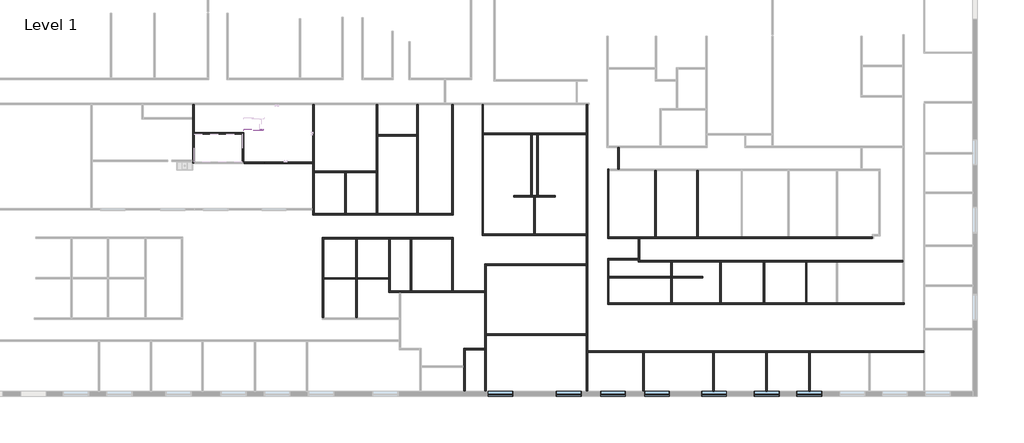
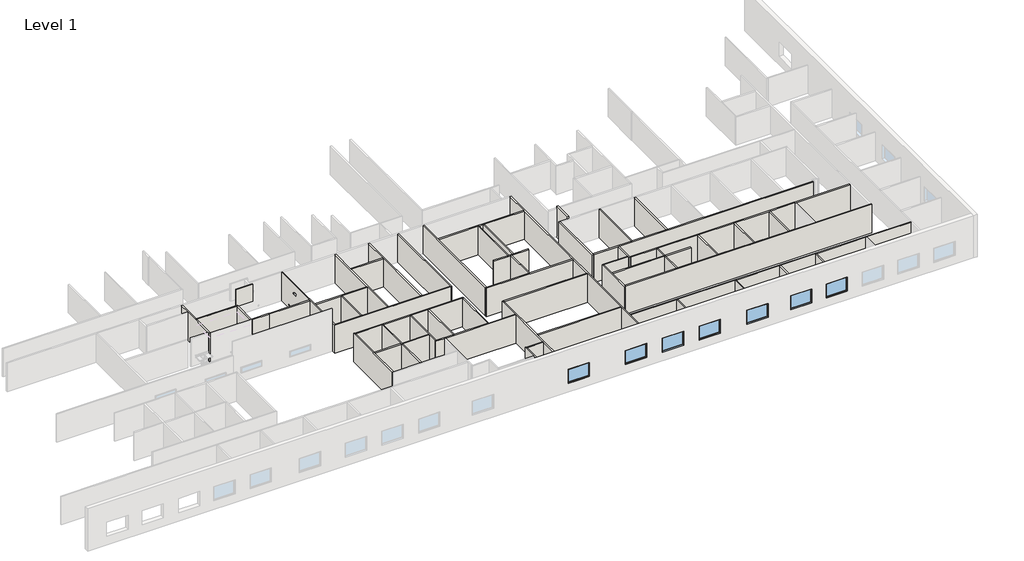
# One storey, part 2 of 4: 55 walls, 7 windows.
"""IFC4 building model written with IfcOpenShell, lengths in millimetres."""

import ifcopenshell
import ifcopenshell.guid

model = None  # the IFC model being written
_history = None  # IfcOwnerHistory: only IFC2X3 demands one
_inside = {}  # id of a spatial element -> (the spatial element, [elements in it])
_under = {}  # id of a project, library or spatial element -> (it, [spatial elements below it])
_declared = {}  # id of a project -> (the project, [libraries it declares])
_typed = {}  # id of a type object -> (the type object, [elements of that type])
_made_of = {}  # id of a material, layer set ... -> (it, [elements and type objects made of it])


def new_model(schema):
    """Start an empty IFC model of exactly this schema.

    Asked for "IFC4X3", IfcOpenShell would pick the latest addendum, in which some entities
    have other attributes; the version numbers below select the first issue.
    IFC2X3 requires an IfcOwnerHistory on every rooted entity: one is made here for all.
    """
    global model, _history
    if schema == "IFC4X3":
        model = ifcopenshell.file(schema_version=(4, 3, 0, 0))
    else:
        model = ifcopenshell.file(schema=schema)
    _inside.clear()
    _under.clear()
    _declared.clear()
    _typed.clear()
    _made_of.clear()
    _history = None
    if model.schema == "IFC2X3":
        org = make("IfcOrganization", Name="unknown")
        user = make(
            "IfcPersonAndOrganization",
            ThePerson=make("IfcPerson", FamilyName="unknown"),
            TheOrganization=org,
        )
        app = make(
            "IfcApplication",
            ApplicationDeveloper=org,
            Version="unknown",
            ApplicationFullName="unknown",
            ApplicationIdentifier="unknown",
        )
        _history = make(
            "IfcOwnerHistory",
            OwningUser=user,
            OwningApplication=app,
            ChangeAction="ADDED",
            CreationDate=0,
        )
    return model


def make(cls, **values):
    """One entity of the class cls with the attributes given. An attribute that is None is left unset."""
    return model.create_entity(
        cls, **{name: value for name, value in values.items() if value is not None}
    )


def rooted(cls, **values):
    """An entity with a GlobalId (a new one), such as an element, a storey or a relation."""
    return make(cls, GlobalId=ifcopenshell.guid.new(), OwnerHistory=_history, **values)


def si_unit(unit_type, name, prefix=None):
    """IfcSIUnit, for example si_unit("LENGTHUNIT", "METRE", prefix="MILLI")."""
    return make("IfcSIUnit", UnitType=unit_type, Prefix=prefix, Name=name)


def assignment(units):
    """IfcUnitAssignment: the units of a project."""
    return None if units is None else make("IfcUnitAssignment", Units=units)


def point(xyz):
    """IfcCartesianPoint."""
    return None if xyz is None else make("IfcCartesianPoint", Coordinates=xyz)


def direction(xyz):
    """IfcDirection."""
    return None if xyz is None else make("IfcDirection", DirectionRatios=xyz)


def frame(location, z_axis=None, x_axis=None):
    """IfcAxis2Placement3D, a coordinate frame: its origin and axes. An axis left out is left unset."""
    return make(
        "IfcAxis2Placement3D",
        Location=point(location),
        Axis=direction(z_axis),
        RefDirection=direction(x_axis),
    )


def origin():
    """The frame at (0, 0, 0) with its axes left unset."""
    return frame((0.0, 0.0, 0.0))


def origin_with_axes():
    """The frame at (0, 0, 0) with the z axis (0, 0, 1) and the x axis (1, 0, 0) written out."""
    return frame((0.0, 0.0, 0.0), z_axis=(0.0, 0.0, 1.0), x_axis=(1.0, 0.0, 0.0))


def place(relative_to, where):
    """IfcLocalPlacement: puts the frame where relative to a parent placement (None: the world)."""
    return make(
        "IfcLocalPlacement", PlacementRelTo=relative_to, RelativePlacement=where
    )


def context(
    kind, dimensions, precision=None, world=None, true_north=None, identifier=None
):
    """IfcGeometricRepresentationContext, for example the 3D "Model" context."""
    return make(
        "IfcGeometricRepresentationContext",
        ContextIdentifier=identifier,
        ContextType=kind,
        CoordinateSpaceDimension=dimensions,
        Precision=precision,
        WorldCoordinateSystem=world,
        TrueNorth=true_north,
    )


def project(units=None, contexts=None):
    """IfcProject with its units and contexts."""
    return rooted(
        "IfcProject",
        Name="project",
        RepresentationContexts=contexts,
        UnitsInContext=assignment(units),
    )


def spatial(cls, under=None, at=None, **own):
    """A site, building, storey or space (cls), placed at a placement, below another one or the project."""
    s = rooted(cls, ObjectPlacement=at, **own)
    if under is not None:
        _under.setdefault(under.id(), (under, []))[1].append(s)
    return s


def polyline(points):
    """IfcPolyline through the points."""
    return make("IfcPolyline", Points=[point(p) for p in points])


def outline(outer, holes=None, kind="AREA"):
    """IfcArbitraryClosedProfileDef: a profile drawn as a closed curve; with holes, ...WithVoids."""
    if holes is None:
        return make("IfcArbitraryClosedProfileDef", ProfileType=kind, OuterCurve=outer)
    return make(
        "IfcArbitraryProfileDefWithVoids",
        ProfileType=kind,
        OuterCurve=outer,
        InnerCurves=holes,
    )


def extrude(swept, where, along, depth):
    """IfcExtrudedAreaSolid: the profile swept, set in the frame where, extruded along a direction by depth."""
    return make(
        "IfcExtrudedAreaSolid",
        SweptArea=swept,
        Position=where,
        ExtrudedDirection=direction(along),
        Depth=depth,
    )


def faces_of(points, faces, orient=None, outer=None):
    """IfcFace entities. A face is a list of loops; a loop is a list of indices into points, from 0.

    orient and outer hold one flag for each loop. By default every Orientation is true, the
    first loop of a face is its IfcFaceOuterBound and the others are IfcFaceBound.
    """
    made = []
    for i, loops in enumerate(faces):
        bounds = []
        for j, loop in enumerate(loops):
            is_outer = j == 0 if outer is None else outer[i][j]
            bounds.append(
                make(
                    "IfcFaceOuterBound" if is_outer else "IfcFaceBound",
                    Bound=make("IfcPolyLoop", Polygon=[points[k] for k in loop]),
                    Orientation=True if orient is None else orient[i][j],
                )
            )
        made.append(make("IfcFace", Bounds=bounds))
    return made


def faceted_brep(points, faces, orient=None, outer=None, voids=None):
    """IfcFacetedBrep: a solid bounded by flat faces; with voids (closed shells), ...WithVoids."""
    shared = [point(p) for p in points]
    hull = make("IfcClosedShell", CfsFaces=faces_of(shared, faces, orient, outer))
    if voids is None:
        return make("IfcFacetedBrep", Outer=hull)
    return make(
        "IfcFacetedBrepWithVoids",
        Outer=hull,
        Voids=[
            make(cls, CfsFaces=faces_of(shared, fs, o, b)) for cls, fs, o, b in voids
        ],
    )


def shape(context_of_items, identifier, shape_type, items):
    """IfcShapeRepresentation: the items that make up one representation, for example the "Body"."""
    return make(
        "IfcShapeRepresentation",
        ContextOfItems=context_of_items,
        RepresentationIdentifier=identifier,
        RepresentationType=shape_type,
        Items=items,
    )


def source(mapping_origin, context_of_items, identifier, shape_type, items):
    """IfcRepresentationMap: a shape defined once, which mapped items show again and again."""
    return make(
        "IfcRepresentationMap",
        MappingOrigin=mapping_origin,
        MappedRepresentation=shape(context_of_items, identifier, shape_type, items),
    )


def transform(
    local_origin,
    x_axis=None,
    y_axis=None,
    z_axis=None,
    scale=None,
    scale2=None,
    scale3=None,
    uniform=True,
):
    """IfcCartesianTransformationOperator3D, or its non-uniform kind. x_axis, y_axis, z_axis: its Axis1, 2, 3."""
    if uniform:
        return make(
            "IfcCartesianTransformationOperator3D",
            Axis1=direction(x_axis),
            Axis2=direction(y_axis),
            LocalOrigin=point(local_origin),
            Scale=scale,
            Axis3=direction(z_axis),
        )
    return make(
        "IfcCartesianTransformationOperator3DnonUniform",
        Axis1=direction(x_axis),
        Axis2=direction(y_axis),
        LocalOrigin=point(local_origin),
        Scale=scale,
        Axis3=direction(z_axis),
        Scale2=scale2,
        Scale3=scale3,
    )


def mapped(mapping_source, mapping_target):
    """IfcMappedItem: shows the shape of a source again, moved by a transform."""
    return make(
        "IfcMappedItem", MappingSource=mapping_source, MappingTarget=mapping_target
    )


def made_of(thing, what):
    """Note that an element or type object is made of a material, layer set ...; save() writes the relation."""
    if what is not None:
        _made_of.setdefault(what.id(), (what, []))[1].append(thing)
    return thing


def element(
    cls,
    number,
    at=None,
    inside=None,
    cuts=None,
    type_object=None,
    material=None,
    context=None,
    identifier="Body",
    shape_type=None,
    held_by="IfcProductDefinitionShape",
    body=None,
    shapes=None,
    **own,
):
    """One element of the class cls, such as IfcWall. Its Tag is "e" and its number.

    at: its placement. inside: the storey or other place that contains it. cuts: it is an
    opening in that element (IfcRelVoidsElement). A single representation is given by context,
    identifier, shape_type and body (its items); several are given by shapes. held_by: the class
    of the entity that holds the representations. save() writes the other relations.
    """
    e = rooted(cls, Tag="e%d" % number, ObjectPlacement=at, **own)
    if body is not None:
        shapes = [shape(context, identifier, shape_type, body)]
    if shapes is not None:
        e.Representation = make(held_by, Representations=shapes)
    if inside is not None:
        _inside.setdefault(inside.id(), (inside, []))[1].append(e)
    if cuts is not None:
        rooted(
            "IfcRelVoidsElement", RelatingBuildingElement=cuts, RelatedOpeningElement=e
        )
    if type_object is not None:
        _typed.setdefault(type_object.id(), (type_object, []))[1].append(e)
    return made_of(e, material)


def aggregate(whole, parts):
    """IfcRelAggregates: a whole, such as a stair, and the parts it consists of."""
    return rooted("IfcRelAggregates", RelatingObject=whole, RelatedObjects=parts)


def save(model, path):
    """Write the relations noted so far, then the file.

    IfcRelAggregates (storeys below a building ...), IfcRelContainedInSpatialStructure (elements
    in a storey), IfcRelDefinesByType, IfcRelAssociatesMaterial and IfcRelDeclares: one each for
    every whole, place, type object, material and project.
    """
    for whole, parts in _under.values():
        aggregate(whole, parts)
    for where, things in _inside.values():
        rooted(
            "IfcRelContainedInSpatialStructure",
            RelatedElements=things,
            RelatingStructure=where,
        )
    for kind, things in _typed.values():
        rooted("IfcRelDefinesByType", RelatedObjects=things, RelatingType=kind)
    for what, things in _made_of.values():
        rooted("IfcRelAssociatesMaterial", RelatedObjects=things, RelatingMaterial=what)
    for by, libraries in _declared.values():
        rooted("IfcRelDeclares", RelatingContext=by, RelatedDefinitions=libraries)
    model.write(path)


def window_d56d71bd(model_context):
    return source(origin(), model_context, "Body", "SweptSolid", [
        extrude(outline(polyline([(990.6, 50.8), (-1066.8, 50.8), (-1066.8, 63.5), (990.6, 63.5), (990.6, 50.8)])), frame((0.0, 0.0, 977.9), z_axis=(0.0, 0.0, 1.0), x_axis=(1.0, 0.0, 0.0)), (0.0, 0.0, 1.0), 1397.0),
        extrude(outline(polyline([(2419.35, -1111.25), (933.45, -1111.25), (933.45, 1035.05), (2419.35, 1035.05), (2419.35, -1111.25)]), holes=[polyline([(2374.9, -1066.8), (2374.9, 990.6), (977.9, 990.6), (977.9, -1066.8), (2374.9, -1066.8)])]), frame((0.0, 34.925, 0.0), z_axis=(0.0, 1.0, 0.0), x_axis=(0.0, 0.0, 1.0)), (0.0, 0.0, 1.0), 44.45),
        extrude(outline(polyline([(2438.4, -1130.3), (914.4, -1130.3), (914.4, 1054.1), (2438.4, 1054.1), (2438.4, -1130.3)]), holes=[polyline([(2406.65, -1098.55), (2406.65, 1022.35), (946.15, 1022.35), (946.15, -1098.55), (2406.65, -1098.55)])]), frame((0.0, -206.375, 0.0), z_axis=(0.0, 1.0, 0.0), x_axis=(0.0, 0.0, 1.0)), (0.0, 0.0, 1.0), 241.3),
        extrude(outline(polyline([(2438.4, 1054.1), (2438.4, -1130.3), (914.4, -1130.3), (914.4, 1054.1), (2438.4, 1054.1)]), holes=[polyline([(2419.35, 1035.05), (933.45, 1035.05), (933.45, -1111.25), (2419.35, -1111.25), (2419.35, 1035.05)])]), frame((0.0, 34.925, 0.0), z_axis=(0.0, 1.0, 0.0), x_axis=(0.0, 0.0, 1.0)), (0.0, 0.0, 1.0), 171.45),
    ])


model = new_model("IFC4")

# Units and contexts
model_context = context("Model", 3, world=origin())
ifc_project = project(units=[si_unit("LENGTHUNIT", "METRE", prefix="MILLI")], contexts=[model_context])

# Site, building, storey
site = spatial("IfcSite", under=ifc_project)
building = spatial("IfcBuilding", under=site)
storey = spatial("IfcBuildingStorey", under=building, Name="Level 1", Elevation=0.0)

# Walls
placement = place(None, origin())
element("IfcWall", 1, ObjectType="Interior - 4 7/8\" Partition (1-hr)", at=placement, inside=storey, context=model_context, shape_type="Brep", body=[
    faceted_brep([(98025.36092, -13962.0306763, 0.0), (95318.3791089, -13962.0306763, 0.0), (95194.5541089, -13962.0306763, 0.0), (91798.8916089, -13962.0306763, 0.0), (91675.0666089, -13962.0306763, 0.0), (89968.3697144, -13962.0306763, 0.0), (89844.5447144, -13962.0306763, 0.0), (89844.5447144, -13962.0306763, 3048.0), (89968.3697144, -13962.0306763, 3048.0), (91675.0666089, -13962.0306763, 3048.0), (91798.8916089, -13962.0306763, 3048.0), (95194.5541089, -13962.0306763, 3048.0), (95318.3791089, -13962.0306763, 3048.0), (98025.36092, -13962.0306763, 3048.0), (89844.5447144, -14085.8556763, 0.0), (90709.8666089, -14085.8556763, 0.0), (90833.6916089, -14085.8556763, 0.0), (98025.36092, -14085.8556763, 0.0), (98025.36092, -14085.8556763, 3048.0), (90833.6916089, -14085.8556763, 3048.0), (90709.8666089, -14085.8556763, 3048.0), (89844.5447144, -14085.8556763, 3048.0)], [[[0, 1, 2, 3, 4, 5, 6, 7, 8, 9, 10, 11, 12, 13]], [[14, 15, 16, 17, 18, 19, 20, 21]], [[6, 5, 4, 3, 2, 1, 0, 17, 16, 15, 14]], [[13, 12, 11, 10, 9, 8, 7, 21, 20, 19, 18]], [[7, 6, 14, 21]], [[0, 13, 18, 17]]]),
])
element("IfcWall", 2, ObjectType="Interior - 4 7/8\" Partition (1-hr)", at=placement, inside=storey, context=model_context, shape_type="Brep", body=[
    faceted_brep([(89968.3697144, -13962.0306763, 0.0), (89968.3697144, -9494.5576294, 0.0), (89968.3697144, -9494.5576294, 3048.0), (89968.3697144, -13962.0306763, 3048.0), (89844.5447144, -13962.0306763, 0.0), (89844.5447144, -13962.0306763, 3048.0), (89844.5447144, -12933.8119327, 3048.0), (89844.5447144, -12809.9869327, 3048.0), (89844.5447144, -9494.5576294, 3048.0), (89844.5447144, -9494.5576294, 0.0), (89844.5447144, -12809.9869327, 0.0), (89844.5447144, -12933.8119327, 0.0)], [[[0, 1, 2, 3]], [[4, 5, 6, 7, 8, 9, 10, 11]], [[1, 0, 4, 11, 10, 9]], [[3, 2, 8, 7, 6, 5]], [[0, 3, 5, 4]], [[2, 1, 9, 8]]]),
])
element("IfcWall", 3, ObjectType="Interior - 4 7/8\" Partition (1-hr)", at=placement, inside=storey, context=model_context, shape_type="Brep", body=[
    faceted_brep([(84269.3791089, -16249.2412361, 0.0), (84269.3791089, -12933.8119327, 0.0), (84269.3791089, -12809.9869327, 0.0), (84269.3791089, -9494.5576294, 0.0), (84269.3791089, -9370.7326294, 0.0), (84269.3791089, -9370.7326294, 3048.0), (84269.3791089, -9494.5576294, 3048.0), (84269.3791089, -12809.9869327, 3048.0), (84269.3791089, -12933.8119327, 3048.0), (84269.3791089, -16249.2412361, 3048.0), (84145.5541089, -16249.2412361, 0.0), (84145.5541089, -16249.2412361, 3048.0), (84145.5541089, -9370.7326294, 3048.0), (84145.5541089, -9370.7326294, 0.0)], [[[0, 1, 2, 3, 4, 5, 6, 7, 8, 9]], [[10, 11, 12, 13]], [[4, 3, 2, 1, 0, 10, 13]], [[9, 8, 7, 6, 5, 12, 11]], [[0, 9, 11, 10]], [[5, 4, 13, 12]]]),
])
element("IfcWall", 4, ObjectType="Interior - 4 7/8\" Partition (1-hr)", at=placement, inside=storey, context=model_context, shape_type="Brep", body=[
    faceted_brep([(84269.3791089, -9494.5576294, 0.0), (86999.7447144, -9494.5576294, 0.0), (87123.5697144, -9494.5576294, 0.0), (89844.5447144, -9494.5576294, 0.0), (89968.3697144, -9494.5576294, 0.0), (91675.0666089, -9494.5576294, 0.0), (91798.8916089, -9494.5576294, 0.0), (95194.5541089, -9494.5576294, 0.0), (95318.3791089, -9494.5576294, 0.0), (95318.3791089, -9494.5576294, 3048.0), (95194.5541089, -9494.5576294, 3048.0), (91798.8916089, -9494.5576294, 3048.0), (91675.0666089, -9494.5576294, 3048.0), (89968.3697144, -9494.5576294, 3048.0), (89844.5447144, -9494.5576294, 3048.0), (87123.5697144, -9494.5576294, 3048.0), (86999.7447144, -9494.5576294, 3048.0), (84269.3791089, -9494.5576294, 3048.0), (95318.3791089, -9370.7326294, 0.0), (84269.3791089, -9370.7326294, 0.0), (84269.3791089, -9370.7326294, 3048.0), (95318.3791089, -9370.7326294, 3048.0)], [[[0, 1, 2, 3, 4, 5, 6, 7, 8, 9, 10, 11, 12, 13, 14, 15, 16, 17]], [[18, 19, 20, 21]], [[8, 7, 6, 5, 4, 3, 2, 1, 0, 19, 18]], [[17, 16, 15, 14, 13, 12, 11, 10, 9, 21, 20]], [[0, 17, 20, 19]], [[9, 8, 18, 21]]]),
])
element("IfcWall", 5, ObjectType="Interior - 4 7/8\" Partition (1-hr)", at=placement, inside=storey, context=model_context, shape_type="SweptSolid", body=[
    extrude(outline(polyline([(95194.5541089, -13962.0306763), (95194.5541089, -9494.5576294), (95318.3791089, -9494.5576294), (95318.3791089, -13962.0306763), (95194.5541089, -13962.0306763)])), origin_with_axes(), (0.0, 0.0, 1.0), 3048.0),
])
element("IfcWall", 6, ObjectType="Interior - 4 7/8\" Partition (1-hr)", at=placement, inside=storey, context=model_context, shape_type="SweptSolid", body=[
    extrude(outline(polyline([(91675.0666089, -13962.0306763), (91675.0666089, -9494.5576294), (91798.8916089, -9494.5576294), (91798.8916089, -13962.0306763), (91675.0666089, -13962.0306763)])), origin_with_axes(), (0.0, 0.0, 1.0), 3048.0),
])
element("IfcWall", 7, ObjectType="Interior - 4 7/8\" Partition (1-hr)", at=placement, inside=storey, context=model_context, shape_type="Brep", body=[
    faceted_brep([(86999.7447144, -9494.5576294, 0.0), (86999.7447144, -12809.9869327, 0.0), (86999.7447144, -12933.8119327, 0.0), (86999.7447144, -16249.2412361, 0.0), (86999.7447144, -16249.2412361, 3048.0), (86999.7447144, -12933.8119327, 3048.0), (86999.7447144, -12809.9869327, 3048.0), (86999.7447144, -9494.5576294, 3048.0), (87123.5697144, -9494.5576294, 0.0), (87123.5697144, -9494.5576294, 3048.0), (87123.5697144, -12809.9869327, 3048.0), (87123.5697144, -12933.8119327, 3048.0), (87123.5697144, -16249.2412361, 3048.0), (87123.5697144, -16249.2412361, 0.0), (87123.5697144, -12933.8119327, 0.0), (87123.5697144, -12809.9869327, 0.0)], [[[0, 1, 2, 3, 4, 5, 6, 7]], [[8, 9, 10, 11, 12, 13, 14, 15]], [[3, 2, 1, 0, 8, 15, 14, 13]], [[7, 6, 5, 4, 12, 11, 10, 9]], [[4, 3, 13, 12]], [[0, 7, 9, 8]]]),
])
element("IfcWall", 8, ObjectType="Interior - 4 7/8\" Partition (1-hr)", at=placement, inside=storey, context=model_context, shape_type="SweptSolid", body=[
    extrude(outline(polyline([(89844.5447144, -12809.9869327), (89844.5447144, -12933.8119327), (87123.5697144, -12933.8119327), (87123.5697144, -12809.9869327), (89844.5447144, -12809.9869327)])), origin_with_axes(), (0.0, 0.0, 1.0), 3048.0),
    extrude(outline(polyline([(84269.3791089, -12933.8119327), (84269.3791089, -12809.9869327), (86999.7447144, -12809.9869327), (86999.7447144, -12933.8119327), (84269.3791089, -12933.8119327)])), origin_with_axes(), (0.0, 0.0, 1.0), 3048.0),
])
element("IfcWall", 9, ObjectType="Interior - 4 7/8\" Partition (1-hr)", at=placement, inside=storey, context=model_context, shape_type="Brep", body=[
    faceted_brep([(95198.8514852, 1981.8368188, 0.0), (95198.8514852, -7317.7381812, 0.0), (95198.8514852, -7441.5631812, 0.0), (95198.8514852, -7441.5631812, 3048.0), (95198.8514852, -7317.7381812, 3048.0), (95198.8514852, 1981.8368188, 3048.0), (95322.6764852, 1981.8368188, 0.0), (95322.6764852, 1981.8368188, 3048.0), (95322.6764852, -7441.5631812, 3048.0), (95322.6764852, -7441.5631812, 0.0)], [[[0, 1, 2, 3, 4, 5]], [[6, 7, 8, 9]], [[2, 1, 0, 6, 9]], [[5, 4, 3, 8, 7]], [[0, 5, 7, 6]], [[3, 2, 9, 8]]]),
])
element("IfcWall", 10, ObjectType="Interior - 4 7/8\" Partition (1-hr)", at=placement, inside=storey, context=model_context, shape_type="Brep", body=[
    faceted_brep([(95198.8514852, -7317.7381812, 0.0), (83460.8764852, -7317.7381812, 0.0), (83337.0514852, -7317.7381812, 0.0), (83337.0514852, -7317.7381812, 3048.0), (83460.8764852, -7317.7381812, 3048.0), (95198.8514852, -7317.7381812, 3048.0), (83337.0514852, -7441.5631812, 0.0), (95198.8514852, -7441.5631812, 0.0), (95198.8514852, -7441.5631812, 3048.0), (83337.0514852, -7441.5631812, 3048.0)], [[[0, 1, 2, 3, 4, 5]], [[6, 7, 8, 9]], [[2, 1, 0, 7, 6]], [[5, 4, 3, 9, 8]], [[0, 5, 8, 7]], [[3, 2, 6, 9]]]),
])
element("IfcWall", 11, ObjectType="Interior - 4 7/8\" Partition (1-hr)", at=placement, inside=storey, context=model_context, shape_type="Brep", body=[
    faceted_brep([(83460.8764852, -7317.7381812, 0.0), (83460.8764852, 1981.8368188, 0.0), (83460.8764852, 1981.8368188, 3048.0), (83460.8764852, -7317.7381812, 3048.0), (83337.0514852, -7317.7381812, 0.0), (83337.0514852, -7317.7381812, 3048.0), (83337.0514852, -3050.1757422, 3048.0), (83337.0514852, -2926.3507422, 3048.0), (83337.0514852, 1981.8368188, 3048.0), (83337.0514852, 1981.8368188, 0.0), (83337.0514852, -2926.3507422, 0.0), (83337.0514852, -3050.1757422, 0.0)], [[[0, 1, 2, 3]], [[4, 5, 6, 7, 8, 9, 10, 11]], [[1, 0, 4, 11, 10, 9]], [[3, 2, 8, 7, 6, 5]], [[0, 3, 5, 4]], [[2, 1, 9, 8]]]),
])
element("IfcWall", 12, ObjectType="Interior - 4 7/8\" Partition (1-hr)", at=placement, inside=storey, context=model_context, shape_type="Brep", body=[
    faceted_brep([(73075.4514852, 1981.8368188, 0.0), (73075.4514852, 886.4618188, 0.0), (73075.4514852, 762.6368188, 0.0), (73075.4514852, -2735.8507422, 0.0), (73075.4514852, -2859.6757422, 0.0), (73075.4514852, -2988.2632422, 0.0), (73075.4514852, -2988.2632422, 3048.0), (73075.4514852, -2859.6757422, 3048.0), (73075.4514852, -2735.8507422, 3048.0), (73075.4514852, 762.6368188, 3048.0), (73075.4514852, 886.4618188, 3048.0), (73075.4514852, 1981.8368188, 3048.0), (73199.2764852, 1981.8368188, 0.0), (73199.2764852, 1981.8368188, 3048.0), (73199.2764852, -415.6239048, 3048.0), (73199.2764852, -539.4489048, 3048.0), (73199.2764852, -2926.3507422, 3048.0), (73199.2764852, -2988.2632422, 3048.0), (73199.2764852, -2988.2632422, 0.0), (73199.2764852, -2926.3507422, 0.0), (73199.2764852, -539.4489048, 0.0), (73199.2764852, -415.6239048, 0.0)], [[[0, 1, 2, 3, 4, 5, 6, 7, 8, 9, 10, 11]], [[12, 13, 14, 15, 16, 17, 18, 19, 20, 21]], [[5, 4, 3, 2, 1, 0, 12, 21, 20, 19, 18]], [[6, 5, 18, 17]], [[11, 10, 9, 8, 7, 6, 17, 16, 15, 14, 13]], [[0, 11, 13, 12]]]),
])
element("IfcWall", 13, ObjectType="Interior - 4 7/8\" Partition (1-hr)", at=placement, inside=storey, context=model_context, shape_type="SweptSolid", body=[
    extrude(outline(polyline([(77291.8514852, -2926.3507422), (77291.8514852, -539.4489048), (77415.6764852, -539.4489048), (77415.6764852, -2926.3507422), (77291.8514852, -2926.3507422)])), origin_with_axes(), (0.0, 0.0, 1.0), 3048.0),
])
element("IfcWall", 14, ObjectType="Interior - 4 7/8\" Partition (1-hr)", at=placement, inside=storey, context=model_context, shape_type="Brep", body=[
    faceted_brep([(77417.2639852, -415.6239048, 0.0), (73199.2764852, -415.6239048, 0.0), (73199.2764852, -415.6239048, 3048.0), (77417.2639852, -415.6239048, 3048.0), (77417.2639852, -539.4489048, 0.0), (77417.2639852, -539.4489048, 3048.0), (77415.6764852, -539.4489048, 3048.0), (77291.8514852, -539.4489048, 3048.0), (73199.2764852, -539.4489048, 3048.0), (73199.2764852, -539.4489048, 0.0), (77291.8514852, -539.4489048, 0.0), (77415.6764852, -539.4489048, 0.0)], [[[0, 1, 2, 3]], [[4, 5, 6, 7, 8, 9, 10, 11]], [[1, 0, 4, 11, 10, 9]], [[3, 2, 8, 7, 6, 5]], [[0, 3, 5, 4]], [[2, 1, 9, 8]]]),
])
element("IfcWall", 15, ObjectType="Interior - 4 7/8\" Partition (1-hr)", at=placement, inside=storey, context=model_context, shape_type="SweptSolid", body=[
    extrude(outline(polyline([(83337.0514852, -3050.1757422), (79120.6514852, -3050.1757422), (79120.6514852, -2926.3507422), (83337.0514852, -2926.3507422), (83337.0514852, -3050.1757422)])), origin_with_axes(), (0.0, 0.0, 1.0), 3048.0),
])
element("IfcWall", 16, ObjectType="Interior - 4 7/8\" Partition (1-hr)", at=placement, inside=storey, context=model_context, shape_type="SweptSolid", body=[
    extrude(outline(polyline([(79182.5639852, -3050.1757422), (77415.6764852, -3050.1757422), (77415.6764852, -2926.3507422), (79182.5639852, -2926.3507422), (79182.5639852, -3050.1757422)])), origin_with_axes(), (0.0, 0.0, 1.0), 3048.0),
])
element("IfcWall", 17, ObjectType="Interior - 4 7/8\" Partition (1-hr)", at=placement, inside=storey, context=model_context, shape_type="Brep", body=[
    faceted_brep([(77415.6764852, -234.6489048, 2743.2), (79120.6514852, -234.6489048, 2743.2), (79120.6514852, -234.6489048, 4572.0), (77415.6764852, -234.6489048, 4572.0), (77415.6764852, -110.8239048, 2743.2), (77415.6764852, -110.8239048, 4572.0), (78815.8514852, -110.8239048, 4572.0), (78939.6764852, -110.8239048, 4572.0), (79120.6514852, -110.8239048, 4572.0), (79120.6514852, -110.8239048, 2743.2), (78939.6764852, -110.8239048, 2743.2), (78815.8514852, -110.8239048, 2743.2)], [[[0, 1, 2, 3]], [[4, 5, 6, 7, 8, 9, 10, 11]], [[1, 0, 4, 11, 10, 9]], [[2, 1, 9, 8]], [[3, 2, 8, 7, 6, 5]], [[0, 3, 5, 4]]]),
])
element("IfcWall", 18, ObjectType="Interior - 4 7/8\" Partition (1-hr)", at=placement, inside=storey, context=model_context, shape_type="Brep", body=[
    faceted_brep([(108519.8686489, -3521.2015997, 0.0), (108519.8686489, -9456.9867961, 0.0), (108519.8686489, -9456.9867961, 3048.0), (108519.8686489, -3521.2015997, 3048.0), (108643.6936489, -3521.2015997, 0.0), (108643.6936489, -3521.2015997, 3048.0), (108643.6936489, -3645.0265997, 3048.0), (108643.6936489, -9333.1617961, 3048.0), (108643.6936489, -9456.9867961, 3048.0), (108643.6936489, -9456.9867961, 0.0), (108643.6936489, -9333.1617961, 0.0), (108643.6936489, -3645.0265997, 0.0)], [[[0, 1, 2, 3]], [[4, 5, 6, 7, 8, 9, 10, 11]], [[1, 0, 4, 11, 10, 9]], [[3, 2, 8, 7, 6, 5]], [[0, 3, 5, 4]], [[2, 1, 9, 8]]]),
])
element("IfcWall", 19, ObjectType="Interior - 4 7/8\" Partition (1-hr)", at=placement, inside=storey, context=model_context, shape_type="Brep", body=[
    faceted_brep([(108643.6936489, -15075.0265997, 0.0), (133865.8936489, -15075.0265997, 0.0), (133865.8936489, -15075.0265997, 3048.0), (108643.6936489, -15075.0265997, 3048.0), (108643.6936489, -14951.2015997, 0.0), (108643.6936489, -14951.2015997, 3048.0), (113933.8980998, -14951.2015997, 3048.0), (114057.7230998, -14951.2015997, 3048.0), (118099.368045, -14951.2015997, 3048.0), (118223.193045, -14951.2015997, 3048.0), (121833.168045, -14951.2015997, 3048.0), (121956.993045, -14951.2015997, 3048.0), (125439.968045, -14951.2015997, 3048.0), (125563.793045, -14951.2015997, 3048.0), (128081.568045, -14951.2015997, 3048.0), (128205.393045, -14951.2015997, 3048.0), (133742.0686489, -14951.2015997, 3048.0), (133865.8936489, -14951.2015997, 3048.0), (133865.8936489, -14951.2015997, 0.0), (133742.0686489, -14951.2015997, 0.0), (128205.393045, -14951.2015997, 0.0), (128081.568045, -14951.2015997, 0.0), (125563.793045, -14951.2015997, 0.0), (125439.968045, -14951.2015997, 0.0), (121956.993045, -14951.2015997, 0.0), (121833.168045, -14951.2015997, 0.0), (118223.193045, -14951.2015997, 0.0), (118099.368045, -14951.2015997, 0.0), (114057.7230998, -14951.2015997, 0.0), (113933.8980998, -14951.2015997, 0.0)], [[[0, 1, 2, 3]], [[4, 5, 6, 7, 8, 9, 10, 11, 12, 13, 14, 15, 16, 17, 18, 19, 20, 21, 22, 23, 24, 25, 26, 27, 28, 29]], [[1, 0, 4, 29, 28, 27, 26, 25, 24, 23, 22, 21, 20, 19, 18]], [[3, 2, 17, 16, 15, 14, 13, 12, 11, 10, 9, 8, 7, 6, 5]], [[0, 3, 5, 4]], [[2, 1, 18, 17]]]),
])
element("IfcWall", 20, ObjectType="Interior - 4 7/8\" Partition (1-hr)", at=placement, inside=storey, context=model_context, shape_type="Brep", body=[
    faceted_brep([(135520.4991283, -19067.1826294, 0.0), (106869.2991283, -19067.1826294, 0.0), (106869.2991283, -19067.1826294, 3048.0), (135520.4991283, -19067.1826294, 3048.0), (135520.4991283, -19191.0076294, 0.0), (135520.4991283, -19191.0076294, 3048.0), (130974.1230998, -19191.0076294, 3048.0), (130850.2980998, -19191.0076294, 3048.0), (125843.3230998, -19191.0076294, 3048.0), (125719.4980998, -19191.0076294, 3048.0), (122160.3230998, -19191.0076294, 3048.0), (122036.4980998, -19191.0076294, 3048.0), (117639.1230998, -19191.0076294, 3048.0), (117515.2980998, -19191.0076294, 3048.0), (111644.7230998, -19191.0076294, 3048.0), (111520.8980998, -19191.0076294, 3048.0), (106869.2991283, -19191.0076294, 3048.0), (106869.2991283, -19191.0076294, 0.0), (111520.8980998, -19191.0076294, 0.0), (111644.7230998, -19191.0076294, 0.0), (117515.2980998, -19191.0076294, 0.0), (117639.1230998, -19191.0076294, 0.0), (122036.4980998, -19191.0076294, 0.0), (122160.3230998, -19191.0076294, 0.0), (125719.4980998, -19191.0076294, 0.0), (125843.3230998, -19191.0076294, 0.0), (130850.2980998, -19191.0076294, 0.0), (130974.1230998, -19191.0076294, 0.0)], [[[0, 1, 2, 3]], [[4, 5, 6, 7, 8, 9, 10, 11, 12, 13, 14, 15, 16, 17, 18, 19, 20, 21, 22, 23, 24, 25, 26, 27]], [[1, 0, 4, 27, 26, 25, 24, 23, 22, 21, 20, 19, 18, 17]], [[2, 1, 17, 16]], [[3, 2, 16, 15, 14, 13, 12, 11, 10, 9, 8, 7, 6, 5]], [[0, 3, 5, 4]]]),
])
element("IfcWall", 21, ObjectType="Interior - 4 7/8\" Partition (1-hr)", at=placement, inside=storey, context=model_context, shape_type="SweptSolid", body=[
    extrude(outline(polyline([(111147.1811489, -11290.4265997), (108643.6936489, -11290.4265997), (108643.6936489, -11166.6015997), (111147.1811489, -11166.6015997), (111147.1811489, -11290.4265997)])), origin_with_axes(), (0.0, 0.0, 1.0), 3048.0),
])
element("IfcWall", 22, ObjectType="Interior - 4 7/8\" Partition (1-hr)", at=placement, inside=storey, context=model_context, shape_type="Brep", body=[
    faceted_brep([(111147.1811489, -9456.9867961, 0.0), (111147.1811489, -11166.6015997, 0.0), (111147.1811489, -11290.4265997, 0.0), (111147.1811489, -11468.2265997, 0.0), (111147.1811489, -11468.2265997, 3048.0), (111147.1811489, -11290.4265997, 3048.0), (111147.1811489, -11166.6015997, 3048.0), (111147.1811489, -9456.9867961, 3048.0), (111271.0061489, -9456.9867961, 0.0), (111271.0061489, -9456.9867961, 3048.0), (111271.0061489, -11344.4015997, 3048.0), (111271.0061489, -11468.2265997, 3048.0), (111271.0061489, -11468.2265997, 0.0), (111271.0061489, -11344.4015997, 0.0)], [[[0, 1, 2, 3, 4, 5, 6, 7]], [[8, 9, 10, 11, 12, 13]], [[3, 2, 1, 0, 8, 13, 12]], [[7, 6, 5, 4, 11, 10, 9]], [[4, 3, 12, 11]], [[0, 7, 9, 8]]]),
])
element("IfcWall", 23, ObjectType="Interior - 4 7/8\" Partition (1-hr)", at=placement, inside=storey, context=model_context, shape_type="Brep", body=[
    faceted_brep([(111271.0061489, -11468.2265997, 0.0), (113933.8980998, -11468.2265997, 0.0), (114057.7230998, -11468.2265997, 0.0), (121833.168045, -11468.2265997, 0.0), (121956.993045, -11468.2265997, 0.0), (125439.968045, -11468.2265997, 0.0), (125563.793045, -11468.2265997, 0.0), (128081.568045, -11468.2265997, 0.0), (128205.393045, -11468.2265997, 0.0), (133742.0686489, -11468.2265997, 0.0), (133742.0686489, -11468.2265997, 3048.0), (128205.393045, -11468.2265997, 3048.0), (128081.568045, -11468.2265997, 3048.0), (125563.793045, -11468.2265997, 3048.0), (125439.968045, -11468.2265997, 3048.0), (121956.993045, -11468.2265997, 3048.0), (121833.168045, -11468.2265997, 3048.0), (118223.193045, -11468.2265997, 3048.0), (118099.368045, -11468.2265997, 3048.0), (114057.7230998, -11468.2265997, 3048.0), (113933.8980998, -11468.2265997, 3048.0), (111271.0061489, -11468.2265997, 3048.0), (111271.0061489, -11344.4015997, 0.0), (111271.0061489, -11344.4015997, 3048.0), (133742.0686489, -11344.4015997, 3048.0), (133742.0686489, -11344.4015997, 0.0)], [[[0, 1, 2, 3, 4, 5, 6, 7, 8, 9, 10, 11, 12, 13, 14, 15, 16, 17, 18, 19, 20, 21]], [[22, 23, 24, 25]], [[9, 8, 7, 6, 5, 4, 3, 2, 1, 0, 22, 25]], [[21, 20, 19, 18, 17, 16, 15, 14, 13, 12, 11, 10, 24, 23]], [[0, 21, 23, 22]], [[10, 9, 25, 24]]]),
])
element("IfcWall", 24, ObjectType="Interior - 4 7/8\" Partition (1-hr)", at=placement, inside=storey, context=model_context, shape_type="SweptSolid", body=[
    extrude(outline(polyline([(125439.968045, -14951.2015997), (125439.968045, -11468.2265997), (125563.793045, -11468.2265997), (125563.793045, -14951.2015997), (125439.968045, -14951.2015997)])), origin_with_axes(), (0.0, 0.0, 1.0), 3048.0),
])
element("IfcWall", 25, ObjectType="Interior - 4 7/8\" Partition (1-hr)", at=placement, inside=storey, context=model_context, shape_type="SweptSolid", body=[
    extrude(outline(polyline([(121833.168045, -14951.2015997), (121833.168045, -11468.2265997), (121956.993045, -11468.2265997), (121956.993045, -14951.2015997), (121833.168045, -14951.2015997)])), origin_with_axes(), (0.0, 0.0, 1.0), 3048.0),
])
element("IfcWall", 26, ObjectType="Interior - 4 7/8\" Partition (1-hr)", at=placement, inside=storey, context=model_context, shape_type="SweptSolid", body=[
    extrude(outline(polyline([(118099.368045, -14951.2015997), (118099.368045, -11468.2265997), (118223.193045, -11468.2265997), (118223.193045, -14951.2015997), (118099.368045, -14951.2015997)])), origin_with_axes(), (0.0, 0.0, 1.0), 3048.0),
])
element("IfcWall", 27, ObjectType="Interior - 4 7/8\" Partition (1-hr)", at=placement, inside=storey, context=model_context, shape_type="Brep", body=[
    faceted_brep([(108643.6936489, -12839.8265997, 0.0), (113933.8980998, -12839.8265997, 0.0), (114057.7230998, -12839.8265997, 0.0), (116658.9811489, -12839.8265997, 0.0), (116658.9811489, -12839.8265997, 3048.0), (114057.7230998, -12839.8265997, 3048.0), (113933.8980998, -12839.8265997, 3048.0), (108643.6936489, -12839.8265997, 3048.0), (108643.6936489, -12716.0015997, 0.0), (108643.6936489, -12716.0015997, 3048.0), (113933.8980998, -12716.0015997, 3048.0), (114057.7230998, -12716.0015997, 3048.0), (116658.9811489, -12716.0015997, 3048.0), (116658.9811489, -12716.0015997, 0.0), (114057.7230998, -12716.0015997, 0.0), (113933.8980998, -12716.0015997, 0.0)], [[[0, 1, 2, 3, 4, 5, 6, 7]], [[8, 9, 10, 11, 12, 13, 14, 15]], [[3, 2, 1, 0, 8, 15, 14, 13]], [[4, 3, 13, 12]], [[7, 6, 5, 4, 12, 11, 10, 9]], [[0, 7, 9, 8]]]),
])
element("IfcWall", 28, ObjectType="Interior - 4 7/8\" Partition (1-hr)", at=placement, inside=storey, context=model_context, shape_type="SweptSolid", body=[
    extrude(outline(polyline([(114057.7230998, -14951.2015997), (113933.8980998, -14951.2015997), (113933.8980998, -12839.8265997), (114057.7230998, -12839.8265997), (114057.7230998, -14951.2015997)])), origin_with_axes(), (0.0, 0.0, 1.0), 3048.0),
    extrude(outline(polyline([(113933.8980998, -11468.2265997), (114057.7230998, -11468.2265997), (114057.7230998, -12716.0015997), (113933.8980998, -12716.0015997), (113933.8980998, -11468.2265997)])), origin_with_axes(), (0.0, 0.0, 1.0), 3048.0),
])
element("IfcWall", 29, ObjectType="Interior - 4 7/8\" Partition (1-hr)", at=placement, inside=storey, context=model_context, shape_type="Brep", body=[
    faceted_brep([(106814.8936489, -22532.6951294, 0.0), (106814.8936489, 1981.8368188, 0.0), (106814.8936489, 1981.8368188, 3048.0), (106814.8936489, -22532.6951294, 3048.0), (106691.0686489, -22532.6951294, 0.0), (106691.0686489, -22532.6951294, 3048.0), (106691.0686489, -17746.3826294, 3048.0), (106691.0686489, -17622.5576294, 3048.0), (106691.0686489, -11777.3826294, 3048.0), (106691.0686489, -11653.5576294, 3048.0), (106691.0686489, -9211.9826294, 3048.0), (106691.0686489, -9088.1576294, 3048.0), (106691.0686489, -572.0469523, 3048.0), (106691.0686489, -448.2219523, 3048.0), (106691.0686489, 1981.8368188, 3048.0), (106691.0686489, 1981.8368188, 0.0), (106691.0686489, -448.2219523, 0.0), (106691.0686489, -572.0469523, 0.0), (106691.0686489, -9088.1576294, 0.0), (106691.0686489, -9211.9826294, 0.0), (106691.0686489, -11653.5576294, 0.0), (106691.0686489, -11777.3826294, 0.0), (106691.0686489, -17622.5576294, 0.0), (106691.0686489, -17746.3826294, 0.0)], [[[0, 1, 2, 3]], [[4, 5, 6, 7, 8, 9, 10, 11, 12, 13, 14, 15, 16, 17, 18, 19, 20, 21, 22, 23]], [[1, 0, 4, 23, 22, 21, 20, 19, 18, 17, 16, 15]], [[3, 2, 14, 13, 12, 11, 10, 9, 8, 7, 6, 5]], [[0, 3, 5, 4]], [[2, 1, 15, 14]]]),
])
element("IfcWall", 30, ObjectType="Interior - 4 7/8\" Partition (1-hr)", at=placement, inside=storey, context=model_context, shape_type="Brep", body=[
    faceted_brep([(98149.18592, -22532.6951294, 0.0), (98149.18592, -17746.3826294, 0.0), (98149.18592, -17622.5576294, 0.0), (98149.18592, -11777.3826294, 0.0), (98149.18592, -11653.5576294, 0.0), (98149.18592, -11653.5576294, 3048.0), (98149.18592, -11777.3826294, 3048.0), (98149.18592, -17622.5576294, 3048.0), (98149.18592, -17746.3826294, 3048.0), (98149.18592, -22532.6951294, 3048.0), (98025.36092, -22532.6951294, 0.0), (98025.36092, -22532.6951294, 3048.0), (98025.36092, -18965.5826294, 3048.0), (98025.36092, -18841.7576294, 3048.0), (98025.36092, -11653.5576294, 3048.0), (98025.36092, -11653.5576294, 0.0), (98025.36092, -18841.7576294, 0.0), (98025.36092, -18965.5826294, 0.0)], [[[0, 1, 2, 3, 4, 5, 6, 7, 8, 9]], [[10, 11, 12, 13, 14, 15, 16, 17]], [[4, 3, 2, 1, 0, 10, 17, 16, 15]], [[9, 8, 7, 6, 5, 14, 13, 12, 11]], [[0, 9, 11, 10]], [[5, 4, 15, 14]]]),
])
element("IfcWall", 31, ObjectType="Interior - 4 7/8\" Partition (1-hr)", at=placement, inside=storey, context=model_context, shape_type="SweptSolid", body=[
    extrude(outline(polyline([(106691.0686489, -11777.3826294), (98149.18592, -11777.3826294), (98149.18592, -11653.5576294), (106691.0686489, -11653.5576294), (106691.0686489, -11777.3826294)])), origin_with_axes(), (0.0, 0.0, 1.0), 3048.0),
])
element("IfcWall", 32, ObjectType="Interior - 4 7/8\" Partition (1-hr)", at=placement, inside=storey, context=model_context, shape_type="Brep", body=[
    faceted_brep([(96345.78592, -22532.6951294, 0.0), (96345.78592, -18965.5826294, 0.0), (96345.78592, -18841.7576294, 0.0), (96345.78592, -18841.7576294, 3048.0), (96345.78592, -18965.5826294, 3048.0), (96345.78592, -22532.6951294, 3048.0), (96221.96092, -22532.6951294, 0.0), (96221.96092, -22532.6951294, 3048.0), (96221.96092, -20486.4076294, 3048.0), (96221.96092, -20362.5826294, 3048.0), (96221.96092, -18841.7576294, 3048.0), (96221.96092, -18841.7576294, 0.0), (96221.96092, -20362.5826294, 0.0), (96221.96092, -20486.4076294, 0.0)], [[[0, 1, 2, 3, 4, 5]], [[6, 7, 8, 9, 10, 11, 12, 13]], [[2, 1, 0, 6, 13, 12, 11]], [[5, 4, 3, 10, 9, 8, 7]], [[0, 5, 7, 6]], [[3, 2, 11, 10]]]),
])
element("IfcWall", 33, ObjectType="Interior - 4 7/8\" Partition (1-hr)", at=placement, inside=storey, context=model_context, shape_type="SweptSolid", body=[
    extrude(outline(polyline([(98025.36092, -18965.5826294), (96345.78592, -18965.5826294), (96345.78592, -18841.7576294), (98025.36092, -18841.7576294), (98025.36092, -18965.5826294)])), origin_with_axes(), (0.0, 0.0, 1.0), 3048.0),
])
element("IfcWall", 34, ObjectType="Interior - 4 7/8\" Partition (1-hr)", at=placement, inside=storey, context=model_context, shape_type="Brep", body=[
    faceted_brep([(106691.0686489, -9088.1576294, 0.0), (102337.7930845, -9088.1576294, 0.0), (102213.9680845, -9088.1576294, 0.0), (97922.6050201, -9088.1576294, 0.0), (97798.7800201, -9088.1576294, 0.0), (97798.7800201, -9088.1576294, 3048.0), (97922.6050201, -9088.1576294, 3048.0), (102213.9680845, -9088.1576294, 3048.0), (102337.7930845, -9088.1576294, 3048.0), (106691.0686489, -9088.1576294, 3048.0), (106691.0686489, -9211.9826294, 0.0), (106691.0686489, -9211.9826294, 3048.0), (97798.7800201, -9211.9826294, 3048.0), (97798.7800201, -9211.9826294, 0.0)], [[[0, 1, 2, 3, 4, 5, 6, 7, 8, 9]], [[10, 11, 12, 13]], [[4, 3, 2, 1, 0, 10, 13]], [[9, 8, 7, 6, 5, 12, 11]], [[0, 9, 11, 10]], [[5, 4, 13, 12]]]),
])
element("IfcWall", 35, ObjectType="Interior - 4 7/8\" Partition (1-hr)", at=placement, inside=storey, context=model_context, shape_type="Brep", body=[
    faceted_brep([(97922.6050201, -9088.1576294, 0.0), (97922.6050201, -572.0469523, 0.0), (97922.6050201, -448.2219523, 0.0), (97922.6050201, 1981.8368188, 0.0), (97922.6050201, 1981.8368188, 3048.0), (97922.6050201, -448.2219523, 3048.0), (97922.6050201, -572.0469523, 3048.0), (97922.6050201, -9088.1576294, 3048.0), (97798.7800201, -9088.1576294, 0.0), (97798.7800201, -9088.1576294, 3048.0), (97798.7800201, 1981.8368188, 3048.0), (97798.7800201, 1981.8368188, 0.0)], [[[0, 1, 2, 3, 4, 5, 6, 7]], [[8, 9, 10, 11]], [[3, 2, 1, 0, 8, 11]], [[7, 6, 5, 4, 10, 9]], [[0, 7, 9, 8]], [[4, 3, 11, 10]]]),
])
element("IfcWall", 36, ObjectType="Interior - 4 7/8\" Partition (1-hr)", at=placement, inside=storey, context=model_context, shape_type="SweptSolid", body=[
    extrude(outline(polyline([(102337.7930845, -5909.9826294), (102337.7930845, -9088.1576294), (102213.9680845, -9088.1576294), (102213.9680845, -5909.9826294), (102337.7930845, -5909.9826294)])), origin_with_axes(), (0.0, 0.0, 1.0), 3048.0),
])
element("IfcWall", 37, ObjectType="Interior - 4 7/8\" Partition (1-hr)", at=placement, inside=storey, context=model_context, shape_type="Brep", body=[
    faceted_brep([(100497.2319539, -5909.9826294, 0.0), (102213.9680845, -5909.9826294, 0.0), (102337.7930845, -5909.9826294, 0.0), (104071.5212769, -5909.9826294, 0.0), (104071.5212769, -5909.9826294, 3048.0), (102337.7930845, -5909.9826294, 3048.0), (102213.9680845, -5909.9826294, 3048.0), (100497.2319539, -5909.9826294, 3048.0), (100497.2319539, -5786.1576294, 0.0), (100497.2319539, -5786.1576294, 3048.0), (101959.9680845, -5786.1576294, 3048.0), (102083.7930845, -5786.1576294, 3048.0), (102473.4048706, -5786.1576294, 3048.0), (102597.2298706, -5786.1576294, 3048.0), (104071.5212769, -5786.1576294, 3048.0), (104071.5212769, -5786.1576294, 0.0), (102597.2298706, -5786.1576294, 0.0), (102473.4048706, -5786.1576294, 0.0), (102083.7930845, -5786.1576294, 0.0), (101959.9680845, -5786.1576294, 0.0)], [[[0, 1, 2, 3, 4, 5, 6, 7]], [[8, 9, 10, 11, 12, 13, 14, 15, 16, 17, 18, 19]], [[3, 2, 1, 0, 8, 19, 18, 17, 16, 15]], [[4, 3, 15, 14]], [[7, 6, 5, 4, 14, 13, 12, 11, 10, 9]], [[0, 7, 9, 8]]]),
])
element("IfcWall", 38, ObjectType="Interior - 4 7/8\" Partition (1-hr)", at=placement, inside=storey, context=model_context, shape_type="SweptSolid", body=[
    extrude(outline(polyline([(102083.7930845, -572.0469523), (102083.7930845, -5786.1576294), (101959.9680845, -5786.1576294), (101959.9680845, -572.0469523), (102083.7930845, -572.0469523)])), origin_with_axes(), (0.0, 0.0, 1.0), 3048.0),
])
element("IfcWall", 39, ObjectType="Interior - 4 7/8\" Partition (1-hr)", at=placement, inside=storey, context=model_context, shape_type="Brep", body=[
    faceted_brep([(97922.6050201, -572.0469523, 0.0), (101959.9680845, -572.0469523, 0.0), (102083.7930845, -572.0469523, 0.0), (102473.4048706, -572.0469523, 0.0), (102597.2298706, -572.0469523, 0.0), (106691.0686489, -572.0469523, 0.0), (106691.0686489, -572.0469523, 3048.0), (102597.2298706, -572.0469523, 3048.0), (102473.4048706, -572.0469523, 3048.0), (102083.7930845, -572.0469523, 3048.0), (101959.9680845, -572.0469523, 3048.0), (97922.6050201, -572.0469523, 3048.0), (97922.6050201, -448.2219523, 0.0), (97922.6050201, -448.2219523, 3048.0), (106691.0686489, -448.2219523, 3048.0), (106691.0686489, -448.2219523, 0.0)], [[[0, 1, 2, 3, 4, 5, 6, 7, 8, 9, 10, 11]], [[12, 13, 14, 15]], [[5, 4, 3, 2, 1, 0, 12, 15]], [[11, 10, 9, 8, 7, 6, 14, 13]], [[0, 11, 13, 12]], [[6, 5, 15, 14]]]),
])
element("IfcWall", 40, ObjectType="Interior - 4 7/8\" Partition (1-hr)", at=placement, inside=storey, context=model_context, shape_type="SweptSolid", body=[
    extrude(outline(polyline([(102473.4048706, -5786.1576294), (102473.4048706, -572.0469523), (102597.2298706, -572.0469523), (102597.2298706, -5786.1576294), (102473.4048706, -5786.1576294)])), origin_with_axes(), (0.0, 0.0, 1.0), 3048.0),
])
element("IfcWall", 41, ObjectType="Interior - 4 7/8\" Partition (1-hr)", at=placement, inside=storey, context=model_context, shape_type="Brep", body=[
    faceted_brep([(88901.5697144, -7317.7381812, 0.0), (88901.5697144, -691.8489048, 0.0), (88901.5697144, -568.0239048, 0.0), (88901.5697144, 1981.8368188, 0.0), (88901.5697144, 1981.8368188, 3048.0), (88901.5697144, -568.0239048, 3048.0), (88901.5697144, -691.8489048, 3048.0), (88901.5697144, -7317.7381812, 3048.0), (88777.7447144, -7317.7381812, 0.0), (88777.7447144, -7317.7381812, 3048.0), (88777.7447144, -3833.4003377, 3048.0), (88777.7447144, -3709.5753377, 3048.0), (88777.7447144, 1981.8368188, 3048.0), (88777.7447144, 1981.8368188, 0.0), (88777.7447144, -3709.5753377, 0.0), (88777.7447144, -3833.4003377, 0.0)], [[[0, 1, 2, 3, 4, 5, 6, 7]], [[8, 9, 10, 11, 12, 13, 14, 15]], [[3, 2, 1, 0, 8, 15, 14, 13]], [[7, 6, 5, 4, 12, 11, 10, 9]], [[0, 7, 9, 8]], [[4, 3, 13, 12]]]),
])
element("IfcWall", 42, ObjectType="Interior - 4 7/8\" Partition (1-hr)", at=placement, inside=storey, context=model_context, shape_type="Brep", body=[
    faceted_brep([(92219.9408081, 1981.8368188, 0.0), (92219.9408081, -568.0239048, 0.0), (92219.9408081, -691.8489048, 0.0), (92219.9408081, -7317.7381812, 0.0), (92219.9408081, -7317.7381812, 3048.0), (92219.9408081, -691.8489048, 3048.0), (92219.9408081, -568.0239048, 3048.0), (92219.9408081, 1981.8368188, 3048.0), (92343.7658081, 1981.8368188, 0.0), (92343.7658081, 1981.8368188, 3048.0), (92343.7658081, -7317.7381812, 3048.0), (92343.7658081, -7317.7381812, 0.0)], [[[0, 1, 2, 3, 4, 5, 6, 7]], [[8, 9, 10, 11]], [[3, 2, 1, 0, 8, 11]], [[7, 6, 5, 4, 10, 9]], [[0, 7, 9, 8]], [[4, 3, 11, 10]]]),
])
element("IfcWall", 43, ObjectType="Interior - 4 7/8\" Partition (1-hr)", at=placement, inside=storey, context=model_context, shape_type="SweptSolid", body=[
    extrude(outline(polyline([(92219.9408081, -691.8489048), (88901.5697144, -691.8489048), (88901.5697144, -568.0239048), (92219.9408081, -568.0239048), (92219.9408081, -691.8489048)])), origin_with_axes(), (0.0, 0.0, 1.0), 3048.0),
])
element("IfcWall", 44, ObjectType="Interior - 4 7/8\" Partition (1-hr)", at=placement, inside=storey, context=model_context, shape_type="Brep", body=[
    faceted_brep([(88777.7447144, -3709.5753377, 0.0), (83460.8764852, -3709.5753377, 0.0), (83460.8764852, -3709.5753377, 3048.0), (88777.7447144, -3709.5753377, 3048.0), (88777.7447144, -3833.4003377, 0.0), (88777.7447144, -3833.4003377, 3048.0), (86181.2230998, -3833.4003377, 3048.0), (86057.3980998, -3833.4003377, 3048.0), (83460.8764852, -3833.4003377, 3048.0), (83460.8764852, -3833.4003377, 0.0), (86057.3980998, -3833.4003377, 0.0), (86181.2230998, -3833.4003377, 0.0)], [[[0, 1, 2, 3]], [[4, 5, 6, 7, 8, 9, 10, 11]], [[1, 0, 4, 11, 10, 9]], [[3, 2, 8, 7, 6, 5]], [[2, 1, 9, 8]], [[0, 3, 5, 4]]]),
])
element("IfcWall", 45, ObjectType="Interior - 4 7/8\" Partition (1-hr)", at=placement, inside=storey, context=model_context, shape_type="SweptSolid", body=[
    extrude(outline(polyline([(86057.3980998, -7317.7381812), (86057.3980998, -3833.4003377), (86181.2230998, -3833.4003377), (86181.2230998, -7317.7381812), (86057.3980998, -7317.7381812)])), origin_with_axes(), (0.0, 0.0, 1.0), 3048.0),
])
element("IfcWall", 46, ObjectType="Interior - 4 7/8\" Partition (1-hr)", at=placement, inside=storey, context=model_context, shape_type="Brep", body=[
    faceted_brep([(131148.9796102, -9333.1617961, 0.0), (128205.393045, -9333.1617961, 0.0), (128081.568045, -9333.1617961, 0.0), (124039.793045, -9333.1617961, 0.0), (123915.968045, -9333.1617961, 0.0), (120051.993045, -9333.1617961, 0.0), (119928.168045, -9333.1617961, 0.0), (116289.0936489, -9333.1617961, 0.0), (116165.2686489, -9333.1617961, 0.0), (112686.1230998, -9333.1617961, 0.0), (112562.2980998, -9333.1617961, 0.0), (108643.6936489, -9333.1617961, 0.0), (108643.6936489, -9333.1617961, 3048.0), (112562.2980998, -9333.1617961, 3048.0), (112686.1230998, -9333.1617961, 3048.0), (116165.2686489, -9333.1617961, 3048.0), (116289.0936489, -9333.1617961, 3048.0), (119928.168045, -9333.1617961, 3048.0), (120051.993045, -9333.1617961, 3048.0), (123915.968045, -9333.1617961, 3048.0), (124039.793045, -9333.1617961, 3048.0), (128081.568045, -9333.1617961, 3048.0), (128205.393045, -9333.1617961, 3048.0), (131148.9796102, -9333.1617961, 3048.0), (131148.9796102, -9456.9867961, 0.0), (131148.9796102, -9456.9867961, 3048.0), (111271.0061489, -9456.9867961, 3048.0), (111147.1811489, -9456.9867961, 3048.0), (108643.6936489, -9456.9867961, 3048.0), (108643.6936489, -9456.9867961, 0.0), (111147.1811489, -9456.9867961, 0.0), (111271.0061489, -9456.9867961, 0.0)], [[[0, 1, 2, 3, 4, 5, 6, 7, 8, 9, 10, 11, 12, 13, 14, 15, 16, 17, 18, 19, 20, 21, 22, 23]], [[24, 25, 26, 27, 28, 29, 30, 31]], [[11, 10, 9, 8, 7, 6, 5, 4, 3, 2, 1, 0, 24, 31, 30, 29]], [[23, 22, 21, 20, 19, 18, 17, 16, 15, 14, 13, 12, 28, 27, 26, 25]], [[0, 23, 25, 24]], [[12, 11, 29, 28]]]),
])
element("IfcWall", 47, ObjectType="Interior - 4 7/8\" Partition (1-hr)", at=placement, inside=storey, context=model_context, shape_type="Brep", body=[
    faceted_brep([(108519.8686489, -11166.6015997, 0.0), (108519.8686489, -15075.0265997, 0.0), (108519.8686489, -15075.0265997, 3048.0), (108519.8686489, -11166.6015997, 3048.0), (108643.6936489, -11166.6015997, 0.0), (108643.6936489, -11166.6015997, 3048.0), (108643.6936489, -11290.4265997, 3048.0), (108643.6936489, -12716.0015997, 3048.0), (108643.6936489, -12839.8265997, 3048.0), (108643.6936489, -14951.2015997, 3048.0), (108643.6936489, -15075.0265997, 3048.0), (108643.6936489, -15075.0265997, 0.0), (108643.6936489, -14951.2015997, 0.0), (108643.6936489, -12839.8265997, 0.0), (108643.6936489, -12716.0015997, 0.0), (108643.6936489, -11290.4265997, 0.0)], [[[0, 1, 2, 3]], [[4, 5, 6, 7, 8, 9, 10, 11, 12, 13, 14, 15]], [[1, 0, 4, 15, 14, 13, 12, 11]], [[3, 2, 10, 9, 8, 7, 6, 5]], [[2, 1, 11, 10]], [[0, 3, 5, 4]]]),
])
element("IfcWall", 48, ObjectType="Interior - 4 7/8\" Partition (1-hr)", at=placement, inside=storey, context=model_context, shape_type="SweptSolid", body=[
    extrude(outline(polyline([(116289.0936489, -3645.0265997), (116289.0936489, -9333.1617961), (116165.2686489, -9333.1617961), (116165.2686489, -3645.0265997), (116289.0936489, -3645.0265997)])), origin_with_axes(), (0.0, 0.0, 1.0), 3048.0),
])
element("IfcWall", 49, ObjectType="Interior - 4 7/8\" Partition (1-hr)", at=placement, inside=storey, context=model_context, shape_type="SweptSolid", body=[
    extrude(outline(polyline([(112562.2980998, -9333.1617961), (112562.2980998, -3645.0265997), (112686.1230998, -3645.0265997), (112686.1230998, -9333.1617961), (112562.2980998, -9333.1617961)])), origin_with_axes(), (0.0, 0.0, 1.0), 3048.0),
])
element("IfcWall", 50, ObjectType="Interior - 4 7/8\" Partition (1-hr)", at=placement, inside=storey, context=model_context, shape_type="SweptSolid", body=[
    extrude(outline(polyline([(106691.0686489, -17746.3826294), (98149.18592, -17746.3826294), (98149.18592, -17622.5576294), (106691.0686489, -17622.5576294), (106691.0686489, -17746.3826294)])), origin_with_axes(), (0.0, 0.0, 1.0), 3048.0),
])
element("IfcWall", 51, ObjectType="Interior - 4 7/8\" Partition (1-hr)", at=placement, inside=storey, context=model_context, shape_type="SweptSolid", body=[
    extrude(outline(polyline([(111644.7230998, -19191.0076294), (111644.7230998, -22532.6951294), (111520.8980998, -22532.6951294), (111520.8980998, -19191.0076294), (111644.7230998, -19191.0076294)])), origin_with_axes(), (0.0, 0.0, 1.0), 3048.0),
])
element("IfcWall", 52, ObjectType="Interior - 4 7/8\" Partition (1-hr)", at=placement, inside=storey, context=model_context, shape_type="SweptSolid", body=[
    extrude(outline(polyline([(117639.1230998, -19191.0076294), (117639.1230998, -22532.6951294), (117515.2980998, -22532.6951294), (117515.2980998, -19191.0076294), (117639.1230998, -19191.0076294)])), origin_with_axes(), (0.0, 0.0, 1.0), 3048.0),
])
element("IfcWall", 53, ObjectType="Interior - 4 7/8\" Partition (1-hr)", at=placement, inside=storey, context=model_context, shape_type="SweptSolid", body=[
    extrude(outline(polyline([(122160.3230998, -19191.0076294), (122160.3230998, -22532.6951294), (122036.4980998, -22532.6951294), (122036.4980998, -19191.0076294), (122160.3230998, -19191.0076294)])), origin_with_axes(), (0.0, 0.0, 1.0), 3048.0),
])
element("IfcWall", 54, ObjectType="Interior - 4 7/8\" Partition (1-hr)", at=placement, inside=storey, context=model_context, shape_type="SweptSolid", body=[
    extrude(outline(polyline([(125843.3230998, -19191.0076294), (125843.3230998, -22532.6951294), (125719.4980998, -22532.6951294), (125719.4980998, -19191.0076294), (125843.3230998, -19191.0076294)])), origin_with_axes(), (0.0, 0.0, 1.0), 3048.0),
])
element("IfcWall", 55, ObjectType="Interior - 4 7/8\" Partition (1-hr)", at=placement, inside=storey, context=model_context, shape_type="SweptSolid", body=[
    extrude(outline(polyline([(109383.4686489, -3521.2015997), (109383.4686489, -1663.8265997), (109507.2936489, -1663.8265997), (109507.2936489, -3521.2015997), (109383.4686489, -3521.2015997)])), frame((0.0, 0.0, -50.4944461), z_axis=(0.0, 0.0, 1.0), x_axis=(1.0, 0.0, 0.0)), (0.0, 0.0, 1.0), 3349.8834491),
])

# Windows
window_shape = window_d56d71bd(model_context)
element("IfcWindow", 56, ObjectType="Fixed : 86\" x 60\"", at=placement, inside=storey, context=model_context, shape_type="MappedRepresentation", body=[
    mapped(window_shape, transform((99327.4428914, -22739.0701294, 0.0), x_axis=(-1.0, 0.0, 0.0), y_axis=(0.0, -1.0, 0.0), z_axis=(0.0, 0.0, 1.0))),
])
element("IfcWindow", 57, ObjectType="Fixed : 86\" x 60\"", at=placement, inside=storey, context=model_context, shape_type="MappedRepresentation", body=[
    mapped(window_shape, transform((105169.4428914, -22739.0701294, 0.0), x_axis=(-1.0, 0.0, 0.0), y_axis=(0.0, -1.0, 0.0), z_axis=(0.0, 0.0, 1.0))),
])
element("IfcWindow", 58, ObjectType="Fixed : 86\" x 60\"", at=placement, inside=storey, context=model_context, shape_type="MappedRepresentation", body=[
    mapped(window_shape, transform((108954.0428914, -22739.0701294, 0.0), x_axis=(-1.0, 0.0, 0.0), y_axis=(0.0, -1.0, 0.0), z_axis=(0.0, 0.0, 1.0))),
])
element("IfcWindow", 59, ObjectType="Fixed : 86\" x 60\"", at=placement, inside=storey, context=model_context, shape_type="MappedRepresentation", body=[
    mapped(window_shape, transform((112713.2428914, -22739.0701294, 0.0), x_axis=(-1.0, 0.0, 0.0), y_axis=(0.0, -1.0, 0.0), z_axis=(0.0, 0.0, 1.0))),
])
element("IfcWindow", 60, ObjectType="Fixed : 86\" x 60\"", at=placement, inside=storey, context=model_context, shape_type="MappedRepresentation", body=[
    mapped(window_shape, transform((117590.0428914, -22739.0701294, 0.0), x_axis=(-1.0, 0.0, 0.0), y_axis=(0.0, -1.0, 0.0), z_axis=(0.0, 0.0, 1.0))),
])
element("IfcWindow", 61, ObjectType="Fixed : 86\" x 60\"", at=placement, inside=storey, context=model_context, shape_type="MappedRepresentation", body=[
    mapped(window_shape, transform((122085.8428914, -22739.0701294, 0.0), x_axis=(-1.0, 0.0, 0.0), y_axis=(0.0, -1.0, 0.0), z_axis=(0.0, 0.0, 1.0))),
])
element("IfcWindow", 62, ObjectType="Fixed : 86\" x 60\"", at=placement, inside=storey, context=model_context, shape_type="MappedRepresentation", body=[
    mapped(window_shape, transform((125718.0428914, -22739.0701294, 0.0), x_axis=(-1.0, 0.0, 0.0), y_axis=(0.0, -1.0, 0.0), z_axis=(0.0, 0.0, 1.0))),
])

save(model, "model.ifc")

# Revit data of these elements
# Project information
#   Organization Name = "Tocci Building Company"
#   Project Issue Date = "Issue Date"
#   Project Status = "PRECONSTRUCTION"
#   Client Name = "DSM"
#   Project Address = "Lexington, MA"
#   Project Name = "DSM LAB RENOVATION"
#   Project Number = "13399"
# Type "Interior - 4 7/8\" Partition (1-hr)"
#   Assembly Code = "C1010145"
#   Width = 0' - 4 7/8"
#   Layers, outside or top first: 0' - 0 5/8" "Gypsum Wall Board" (function 5); 0' - 3 5/8" "Metal Stud Layer" (function 1); 0' - 0 5/8" "Gypsum Wall Board" (function 5)
# Type "Fixed : 86\" x 60\""
#   Type Mark = "19"
#   Construction Type Id = "GSP4R"
#   Assembly Code = "B2020100"
#   Analytic Construction = "1/8 in Pilkington single glazing"
#   Visual Light Transmittance = 0.9
#   Solar Heat Gain Coefficient = 0.78
#   Heat Transfer Coefficient (U) = 3.6886 W/(m²·K)
#   Height = 5' - 0"
#   Default Sill Height = 3' - 0"
#   Width = 7' - 2"
#   Window Inset = 0' - 5"
#   Glass Pane Material = Glass
#   Sash Material = Sash
#   Wall Closure = (empty or 0)
# Elements 1, 3, 4, 9, 10, 15 (IfcWall, "Interior - 4 7/8\" Partition (1-hr)")
#   Top Offset = 0' - 0"
#   Base Offset = 0' - 0"
#   Unconnected Height = 10' - 0"
#   wall height = 10' - 0"
#   Phase Created = 01 - Existing
#   Base Constraint = Level 1
#   Materials on its faces: "Gypsum Wall Board", "Default Wall"
# Elements 2, 5, 6, 7, 8, 11, 12, 13, 14 (IfcWall, "Interior - 4 7/8\" Partition (1-hr)")
#   Top Offset = 0' - 0"
#   Base Offset = 0' - 0"
#   Unconnected Height = 10' - 0"
#   wall height = 10' - 0"
#   Phase Created = 01 - Existing
#   Base Constraint = Level 1
#   Materials on its faces: "Default Wall", "Gypsum Wall Board"
# Elements 16, 20, 21, 23, 24, 25, 26, 27, 28, 29, 31, 33, 35, 36, 37, 38, 39, 40, 41, 42, 43, 44, 45, 46, 48, 49, 50, 51, 52, 53, 54 (IfcWall, "Interior - 4 7/8\" Partition (1-hr)")
#   Top Offset = 0' - 0"
#   Base Offset = 0' - 0"
#   Unconnected Height = 10' - 0"
#   wall height = 10' - 0"
#   Phase Created = 03 - Project Completion
#   Base Constraint = Level 1
#   Materials on its faces: "Default Wall", "Gypsum Wall Board"
